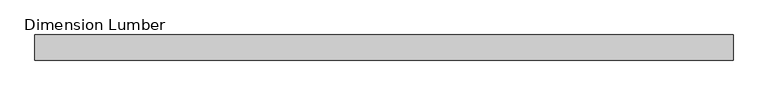
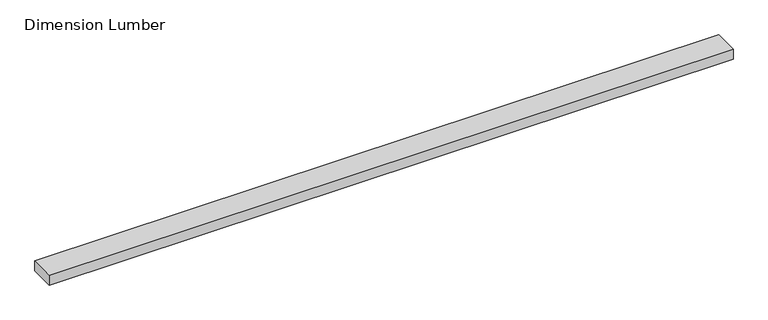
"""IFC4 building model written with IfcOpenShell, lengths in millimetres: beam geometry, Dimension Lumber : Top Supporting Lumbers."""

import ifcopenshell
import ifcopenshell.guid

model = None  # the IFC model being written
_history = None  # IfcOwnerHistory: only IFC2X3 demands one
_inside = {}  # id of a spatial element -> (the spatial element, [elements in it])
_under = {}  # id of a project, library or spatial element -> (it, [spatial elements below it])
_declared = {}  # id of a project -> (the project, [libraries it declares])
_typed = {}  # id of a type object -> (the type object, [elements of that type])
_made_of = {}  # id of a material, layer set ... -> (it, [elements and type objects made of it])


def new_model(schema):
    """Start an empty IFC model of exactly this schema.

    Asked for "IFC4X3", IfcOpenShell would pick the latest addendum, in which some entities
    have other attributes; the version numbers below select the first issue.
    IFC2X3 requires an IfcOwnerHistory on every rooted entity: one is made here for all.
    """
    global model, _history
    if schema == "IFC4X3":
        model = ifcopenshell.file(schema_version=(4, 3, 0, 0))
    else:
        model = ifcopenshell.file(schema=schema)
    _inside.clear()
    _under.clear()
    _declared.clear()
    _typed.clear()
    _made_of.clear()
    _history = None
    if model.schema == "IFC2X3":
        org = make("IfcOrganization", Name="unknown")
        user = make(
            "IfcPersonAndOrganization",
            ThePerson=make("IfcPerson", FamilyName="unknown"),
            TheOrganization=org,
        )
        app = make(
            "IfcApplication",
            ApplicationDeveloper=org,
            Version="unknown",
            ApplicationFullName="unknown",
            ApplicationIdentifier="unknown",
        )
        _history = make(
            "IfcOwnerHistory",
            OwningUser=user,
            OwningApplication=app,
            ChangeAction="ADDED",
            CreationDate=0,
        )
    return model


def make(cls, **values):
    """One entity of the class cls with the attributes given. An attribute that is None is left unset."""
    return model.create_entity(
        cls, **{name: value for name, value in values.items() if value is not None}
    )


def rooted(cls, **values):
    """An entity with a GlobalId (a new one), such as an element, a storey or a relation."""
    return make(cls, GlobalId=ifcopenshell.guid.new(), OwnerHistory=_history, **values)


def si_unit(unit_type, name, prefix=None):
    """IfcSIUnit, for example si_unit("LENGTHUNIT", "METRE", prefix="MILLI")."""
    return make("IfcSIUnit", UnitType=unit_type, Prefix=prefix, Name=name)


def assignment(units):
    """IfcUnitAssignment: the units of a project."""
    return None if units is None else make("IfcUnitAssignment", Units=units)


def point(xyz):
    """IfcCartesianPoint."""
    return None if xyz is None else make("IfcCartesianPoint", Coordinates=xyz)


def direction(xyz):
    """IfcDirection."""
    return None if xyz is None else make("IfcDirection", DirectionRatios=xyz)


def frame(location, z_axis=None, x_axis=None):
    """IfcAxis2Placement3D, a coordinate frame: its origin and axes. An axis left out is left unset."""
    return make(
        "IfcAxis2Placement3D",
        Location=point(location),
        Axis=direction(z_axis),
        RefDirection=direction(x_axis),
    )


def origin():
    """The frame at (0, 0, 0) with its axes left unset."""
    return frame((0.0, 0.0, 0.0))


def place(relative_to, where):
    """IfcLocalPlacement: puts the frame where relative to a parent placement (None: the world)."""
    return make(
        "IfcLocalPlacement", PlacementRelTo=relative_to, RelativePlacement=where
    )


def context(
    kind, dimensions, precision=None, world=None, true_north=None, identifier=None
):
    """IfcGeometricRepresentationContext, for example the 3D "Model" context."""
    return make(
        "IfcGeometricRepresentationContext",
        ContextIdentifier=identifier,
        ContextType=kind,
        CoordinateSpaceDimension=dimensions,
        Precision=precision,
        WorldCoordinateSystem=world,
        TrueNorth=true_north,
    )


def project(units=None, contexts=None):
    """IfcProject with its units and contexts."""
    return rooted(
        "IfcProject",
        Name="project",
        RepresentationContexts=contexts,
        UnitsInContext=assignment(units),
    )


def spatial(cls, under=None, at=None, **own):
    """A site, building, storey or space (cls), placed at a placement, below another one or the project."""
    s = rooted(cls, ObjectPlacement=at, **own)
    if under is not None:
        _under.setdefault(under.id(), (under, []))[1].append(s)
    return s


def polyline(points):
    """IfcPolyline through the points."""
    return make("IfcPolyline", Points=[point(p) for p in points])


def outline(outer, holes=None, kind="AREA"):
    """IfcArbitraryClosedProfileDef: a profile drawn as a closed curve; with holes, ...WithVoids."""
    if holes is None:
        return make("IfcArbitraryClosedProfileDef", ProfileType=kind, OuterCurve=outer)
    return make(
        "IfcArbitraryProfileDefWithVoids",
        ProfileType=kind,
        OuterCurve=outer,
        InnerCurves=holes,
    )


def extrude(swept, where, along, depth):
    """IfcExtrudedAreaSolid: the profile swept, set in the frame where, extruded along a direction by depth."""
    return make(
        "IfcExtrudedAreaSolid",
        SweptArea=swept,
        Position=where,
        ExtrudedDirection=direction(along),
        Depth=depth,
    )


def shape(context_of_items, identifier, shape_type, items):
    """IfcShapeRepresentation: the items that make up one representation, for example the "Body"."""
    return make(
        "IfcShapeRepresentation",
        ContextOfItems=context_of_items,
        RepresentationIdentifier=identifier,
        RepresentationType=shape_type,
        Items=items,
    )


def source(mapping_origin, context_of_items, identifier, shape_type, items):
    """IfcRepresentationMap: a shape defined once, which mapped items show again and again."""
    return make(
        "IfcRepresentationMap",
        MappingOrigin=mapping_origin,
        MappedRepresentation=shape(context_of_items, identifier, shape_type, items),
    )


def transform(
    local_origin,
    x_axis=None,
    y_axis=None,
    z_axis=None,
    scale=None,
    scale2=None,
    scale3=None,
    uniform=True,
):
    """IfcCartesianTransformationOperator3D, or its non-uniform kind. x_axis, y_axis, z_axis: its Axis1, 2, 3."""
    if uniform:
        return make(
            "IfcCartesianTransformationOperator3D",
            Axis1=direction(x_axis),
            Axis2=direction(y_axis),
            LocalOrigin=point(local_origin),
            Scale=scale,
            Axis3=direction(z_axis),
        )
    return make(
        "IfcCartesianTransformationOperator3DnonUniform",
        Axis1=direction(x_axis),
        Axis2=direction(y_axis),
        LocalOrigin=point(local_origin),
        Scale=scale,
        Axis3=direction(z_axis),
        Scale2=scale2,
        Scale3=scale3,
    )


def mapped(mapping_source, mapping_target):
    """IfcMappedItem: shows the shape of a source again, moved by a transform."""
    return make(
        "IfcMappedItem", MappingSource=mapping_source, MappingTarget=mapping_target
    )


def made_of(thing, what):
    """Note that an element or type object is made of a material, layer set ...; save() writes the relation."""
    if what is not None:
        _made_of.setdefault(what.id(), (what, []))[1].append(thing)
    return thing


def element(
    cls,
    number,
    at=None,
    inside=None,
    cuts=None,
    type_object=None,
    material=None,
    context=None,
    identifier="Body",
    shape_type=None,
    held_by="IfcProductDefinitionShape",
    body=None,
    shapes=None,
    **own,
):
    """One element of the class cls, such as IfcWall. Its Tag is "e" and its number.

    at: its placement. inside: the storey or other place that contains it. cuts: it is an
    opening in that element (IfcRelVoidsElement). A single representation is given by context,
    identifier, shape_type and body (its items); several are given by shapes. held_by: the class
    of the entity that holds the representations. save() writes the other relations.
    """
    e = rooted(cls, Tag="e%d" % number, ObjectPlacement=at, **own)
    if body is not None:
        shapes = [shape(context, identifier, shape_type, body)]
    if shapes is not None:
        e.Representation = make(held_by, Representations=shapes)
    if inside is not None:
        _inside.setdefault(inside.id(), (inside, []))[1].append(e)
    if cuts is not None:
        rooted(
            "IfcRelVoidsElement", RelatingBuildingElement=cuts, RelatedOpeningElement=e
        )
    if type_object is not None:
        _typed.setdefault(type_object.id(), (type_object, []))[1].append(e)
    return made_of(e, material)


def aggregate(whole, parts):
    """IfcRelAggregates: a whole, such as a stair, and the parts it consists of."""
    return rooted("IfcRelAggregates", RelatingObject=whole, RelatedObjects=parts)


def save(model, path):
    """Write the relations noted so far, then the file.

    IfcRelAggregates (storeys below a building ...), IfcRelContainedInSpatialStructure (elements
    in a storey), IfcRelDefinesByType, IfcRelAssociatesMaterial and IfcRelDeclares: one each for
    every whole, place, type object, material and project.
    """
    for whole, parts in _under.values():
        aggregate(whole, parts)
    for where, things in _inside.values():
        rooted(
            "IfcRelContainedInSpatialStructure",
            RelatedElements=things,
            RelatingStructure=where,
        )
    for kind, things in _typed.values():
        rooted("IfcRelDefinesByType", RelatedObjects=things, RelatingType=kind)
    for what, things in _made_of.values():
        rooted("IfcRelAssociatesMaterial", RelatedObjects=things, RelatingMaterial=what)
    for by, libraries in _declared.values():
        rooted("IfcRelDeclares", RelatingContext=by, RelatedDefinitions=libraries)
    model.write(path)


def dimension_lumber_8a2991dc(model_context):
    return source(origin(), model_context, "Body", "SweptSolid", [
        extrude(outline(polyline([(1279.525, 44.45), (1279.525, -44.45), (-1190.625, -44.45), (-1190.625, 44.45), (1279.525, 44.45)])), frame((0.0, 0.0, -19.05), z_axis=(0.0, 0.0, 1.0), x_axis=(1.0, 0.0, 0.0)), (0.0, 0.0, 1.0), 38.1),
    ])


if __name__ == "__main__":
    model = new_model("IFC4")
    model_context = context("Model", 3, world=origin())
    ifc_project = project(units=[si_unit("LENGTHUNIT", "METRE", prefix="MILLI")], contexts=[model_context])
    site = spatial("IfcSite", under=ifc_project)
    building = spatial("IfcBuilding", under=site)
    placement = place(None, origin())
    dimension_lumber_shape = dimension_lumber_8a2991dc(model_context)
    element("IfcBeam", 1, ObjectType="Dimension Lumber : Top Supporting Lumbers", at=placement, inside=building, context=model_context, shape_type="MappedRepresentation", body=[
        mapped(dimension_lumber_shape, transform((0.0, 0.0, 0.0), x_axis=(1.0, 0.0, 0.0), y_axis=(0.0, 1.0, 0.0), z_axis=(0.0, 0.0, 1.0))),
    ])
    save(model, "model.ifc")

# Revit data of these elements
# Type "Dimension Lumber : Top Supporting Lumbers"
#   Assembly Code = "B10"
#   A = 0.0364583 SF
#   Length [instance default] = 5' - 0"
#   b = 0' - 3 1/2"
#   d = 0' - 1 1/2"
#   Structural Material [instance default] = Softwood, Lumber
# Element 1 (IfcBeam, "Dimension Lumber : Top Supporting Lumbers")
#   Structural Material = Douglas Fir #2
#   Materials on its faces: "Douglas Fir #2"
# Materials
#   "Softwood, Lumber": class "Wood", colour RGB 223 192 134, transparency 0, Description = "Pinus Echinata", Cost = 0
#   "Douglas Fir #2": class "Wood", colour RGB 223 192 134, transparency 0, Description = "Pinus Echinata", Cost = 0
